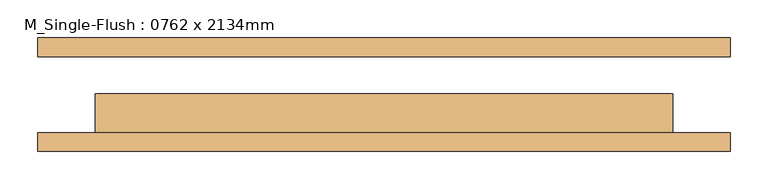
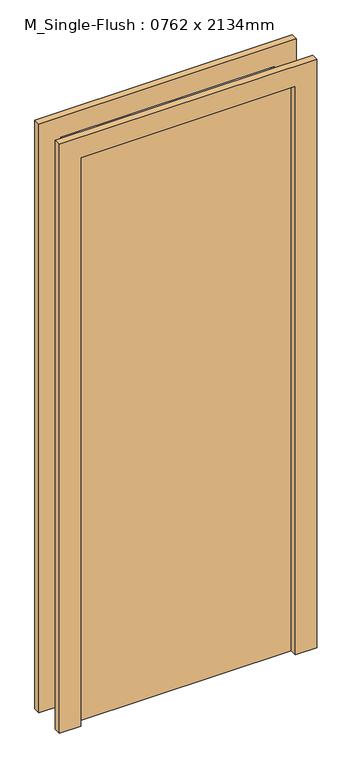
"""IFC4 building model written with IfcOpenShell, lengths in millimetres: door geometry, M_Single-Flush : 0762 x 2134mm."""

from ifc_helpers import new_model, si_unit, frame, origin, origin_with_axes, place, context, project, spatial, polyline, outline, extrude, source, transform, mapped, element, save


def m_single_flush_0762_x_2134mm_2f099e9c(model_context):
    return source(origin(), model_context, "Body", "SweptSolid", [
        extrude(outline(polyline([(2210.0, -457.0), (0.0, -457.0), (0.0, -381.0), (2134.0, -381.0), (2134.0, 381.0), (0.0, 381.0), (0.0, 457.0), (2210.0, 457.0), (2210.0, -457.0)])), frame((0.0, -75.0, 0.0), z_axis=(0.0, 1.0, 0.0), x_axis=(0.0, 0.0, 1.0)), (0.0, 0.0, 1.0), 25.0),
        extrude(outline(polyline([(2210.0, 457.0), (2210.0, -457.0), (0.0, -457.0), (0.0, -381.0), (2134.0, -381.0), (2134.0, 381.0), (0.0, 381.0), (0.0, 457.0), (2210.0, 457.0)])), frame((0.0, 50.0, 0.0), z_axis=(0.0, 1.0, 0.0), x_axis=(0.0, 0.0, 1.0)), (0.0, 0.0, 1.0), 25.0),
        extrude(outline(polyline([(381.0, 1.0), (381.0, -50.0), (-381.0, -50.0), (-381.0, 1.0), (381.0, 1.0)])), origin_with_axes(), (0.0, 0.0, 1.0), 2134.0),
    ])


if __name__ == "__main__":
    model = new_model("IFC4")
    model_context = context("Model", 3, world=origin())
    ifc_project = project(units=[si_unit("LENGTHUNIT", "METRE", prefix="MILLI")], contexts=[model_context])
    site = spatial("IfcSite", under=ifc_project)
    building = spatial("IfcBuilding", under=site)
    placement = place(None, origin())
    m_single_flush_0762_x_2134mm_shape = m_single_flush_0762_x_2134mm_2f099e9c(model_context)
    element("IfcDoor", 1, ObjectType="M_Single-Flush : 0762 x 2134mm", at=placement, inside=building, context=model_context, shape_type="MappedRepresentation", body=[
        mapped(m_single_flush_0762_x_2134mm_shape, transform((0.0, 0.0, 0.0), x_axis=(1.0, 0.0, 0.0), y_axis=(0.0, 1.0, 0.0), z_axis=(0.0, 0.0, 1.0))),
    ])
    save(model, "model.ifc")

# Revit data of these elements
# Type "M_Single-Flush : 0762 x 2134mm"
#   Type Mark = "18"
#   Thickness = 5.1 cm
#   Height = 213.4 cm
#   Trim Projection Ext = 2.5 cm
#   Trim Projection Int = 2.5 cm
#   Trim Width = 7.6 cm
#   Width = 76.2 cm
#   Door Material = Door - Panel
#   Frame Material = Door - Frame
#   Function = (empty or 0)
#   Wall Closure = (empty or 0)
# Element 1 (IfcDoor, "M_Single-Flush : 0762 x 2134mm")
#   Materials on its faces: "Door - Frame", "Door - Panel"
# Materials
#   "Door - Panel": class "Wood", colour RGB 114 82 51, transparency 0
#   "Door - Frame": class "Miscellaneous", colour RGB 153 76 43, transparency 0
